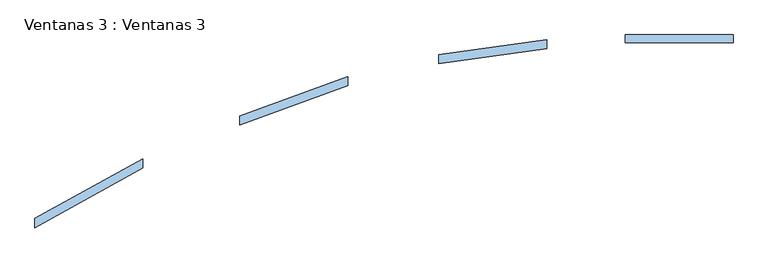
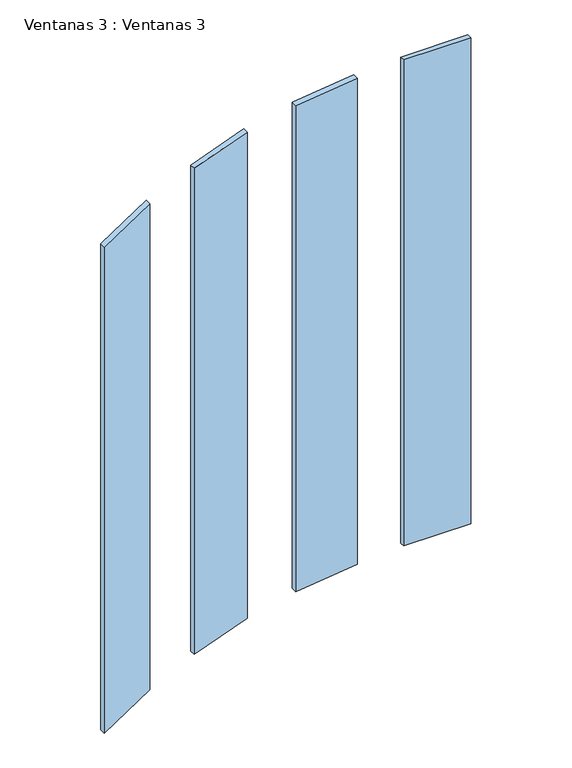
"""IFC4 building model written with IfcOpenShell, lengths in millimetres: window geometry, Ventanas 3 : Ventanas 3."""

from ifc_helpers import new_model, si_unit, frame, origin, place, context, project, spatial, polyline, outline, extrude, source, transform, mapped, element, save


def ventanas_3_ventanas_3_2eb13cfc(model_context):
    return source(origin(), model_context, "Body", "SweptSolid", [
        extrude(outline(polyline([(-9135.7497434, 10735.8910052), (-9135.7497434, 10752.9012379), (-8901.2450065, 10752.9012379), (-8901.2450065, 10735.8910052), (-9135.7497434, 10735.8910052)])), frame((0.0, 0.0, 6206.6549752), z_axis=(0.0, 0.0, 1.0), x_axis=(1.0, 0.0, 0.0)), (0.0, 0.0, 1.0), 1799.693024),
        extrude(outline(polyline([(-9540.4851586, 10709.9437464), (-9305.9804216, 10742.9012379), (-9305.9804216, 10722.9012379), (-9540.4851586, 10689.9437464), (-9540.4851586, 10709.9437464)])), frame((0.0, 0.0, 6206.6549752), z_axis=(0.0, 0.0, 1.0), x_axis=(1.0, 0.0, 0.0)), (0.0, 0.0, 1.0), 1799.693024),
        extrude(outline(polyline([(-9972.8335676, 10576.7858875), (-9738.3288307, 10662.1386316), (-9738.3288307, 10642.1386316), (-9972.8335676, 10556.7858875), (-9972.8335676, 10576.7858875)])), frame((0.0, 0.0, 6206.6549752), z_axis=(0.0, 0.0, 1.0), x_axis=(1.0, 0.0, 0.0)), (0.0, 0.0, 1.0), 1799.693024),
        extrude(outline(polyline([(-10417.4239131, 10353.2616498), (-10182.9191742, 10483.2497491), (-10182.9191742, 10463.2497491), (-10417.4239131, 10333.2616498), (-10417.4239131, 10353.2616498)])), frame((0.0, 0.0, 6206.6549752), z_axis=(0.0, 0.0, 1.0), x_axis=(1.0, 0.0, 0.0)), (0.0, 0.0, 1.0), 1799.693024),
    ])


if __name__ == "__main__":
    model = new_model("IFC4")
    model_context = context("Model", 3, world=origin())
    ifc_project = project(units=[si_unit("LENGTHUNIT", "METRE", prefix="MILLI")], contexts=[model_context])
    site = spatial("IfcSite", under=ifc_project)
    building = spatial("IfcBuilding", under=site)
    placement = place(None, origin())
    ventanas_3_ventanas_3_shape = ventanas_3_ventanas_3_2eb13cfc(model_context)
    element("IfcWindow", 1, ObjectType="Ventanas 3 : Ventanas 3", at=placement, inside=building, context=model_context, shape_type="MappedRepresentation", body=[
        mapped(ventanas_3_ventanas_3_shape, transform((0.0, 0.0, 0.0), x_axis=(1.0, 0.0, 0.0), y_axis=(0.0, 1.0, 0.0), z_axis=(0.0, 0.0, 1.0))),
    ])
    save(model, "model.ifc")

# Revit data of these elements
# Type "Ventanas 3 : Ventanas 3"
#   Type Mark = "29"
# Element 1 (IfcWindow, "Ventanas 3 : Ventanas 3")
#   Materials on its faces: "VIDRIO"
# Materials
#   "VIDRIO": class "Genérico", colour RGB 120 120 120, transparency 0, Cost = 0
